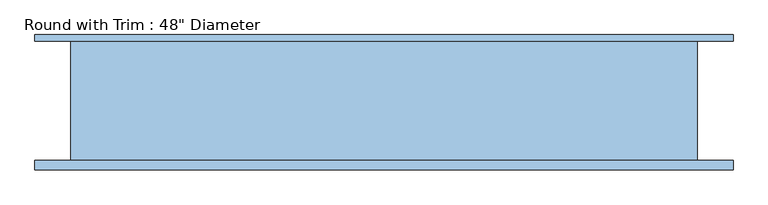
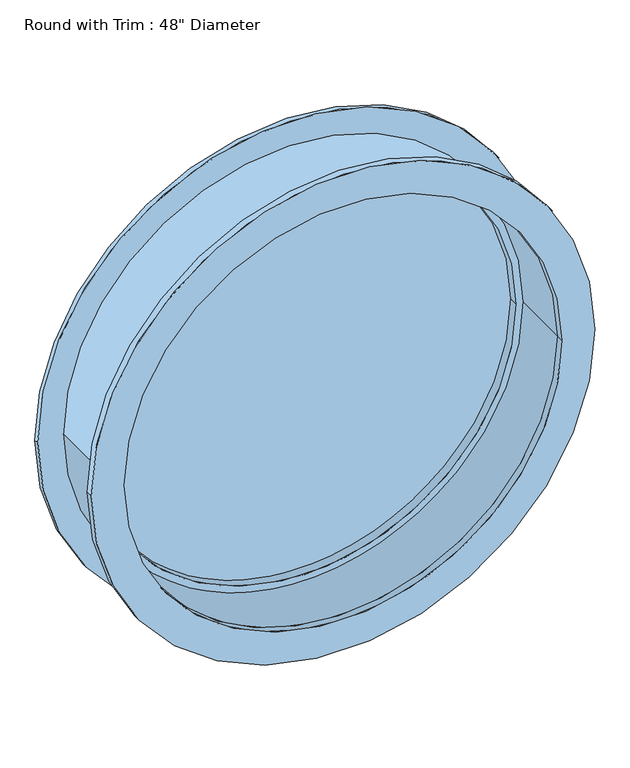
"""IFC4 building model written with IfcOpenShell, lengths in millimetres: window geometry."""

import ifcopenshell
import ifcopenshell.guid

model = None  # the IFC model being written
_history = None  # IfcOwnerHistory: only IFC2X3 demands one
_inside = {}  # id of a spatial element -> (the spatial element, [elements in it])
_under = {}  # id of a project, library or spatial element -> (it, [spatial elements below it])
_declared = {}  # id of a project -> (the project, [libraries it declares])
_typed = {}  # id of a type object -> (the type object, [elements of that type])
_made_of = {}  # id of a material, layer set ... -> (it, [elements and type objects made of it])


def new_model(schema):
    """Start an empty IFC model of exactly this schema.

    Asked for "IFC4X3", IfcOpenShell would pick the latest addendum, in which some entities
    have other attributes; the version numbers below select the first issue.
    IFC2X3 requires an IfcOwnerHistory on every rooted entity: one is made here for all.
    """
    global model, _history
    if schema == "IFC4X3":
        model = ifcopenshell.file(schema_version=(4, 3, 0, 0))
    else:
        model = ifcopenshell.file(schema=schema)
    _inside.clear()
    _under.clear()
    _declared.clear()
    _typed.clear()
    _made_of.clear()
    _history = None
    if model.schema == "IFC2X3":
        org = make("IfcOrganization", Name="unknown")
        user = make(
            "IfcPersonAndOrganization",
            ThePerson=make("IfcPerson", FamilyName="unknown"),
            TheOrganization=org,
        )
        app = make(
            "IfcApplication",
            ApplicationDeveloper=org,
            Version="unknown",
            ApplicationFullName="unknown",
            ApplicationIdentifier="unknown",
        )
        _history = make(
            "IfcOwnerHistory",
            OwningUser=user,
            OwningApplication=app,
            ChangeAction="ADDED",
            CreationDate=0,
        )
    return model


def make(cls, **values):
    """One entity of the class cls with the attributes given. An attribute that is None is left unset."""
    return model.create_entity(
        cls, **{name: value for name, value in values.items() if value is not None}
    )


def rooted(cls, **values):
    """An entity with a GlobalId (a new one), such as an element, a storey or a relation."""
    return make(cls, GlobalId=ifcopenshell.guid.new(), OwnerHistory=_history, **values)


def si_unit(unit_type, name, prefix=None):
    """IfcSIUnit, for example si_unit("LENGTHUNIT", "METRE", prefix="MILLI")."""
    return make("IfcSIUnit", UnitType=unit_type, Prefix=prefix, Name=name)


def assignment(units):
    """IfcUnitAssignment: the units of a project."""
    return None if units is None else make("IfcUnitAssignment", Units=units)


def point(xyz):
    """IfcCartesianPoint."""
    return None if xyz is None else make("IfcCartesianPoint", Coordinates=xyz)


def direction(xyz):
    """IfcDirection."""
    return None if xyz is None else make("IfcDirection", DirectionRatios=xyz)


def frame(location, z_axis=None, x_axis=None):
    """IfcAxis2Placement3D, a coordinate frame: its origin and axes. An axis left out is left unset."""
    return make(
        "IfcAxis2Placement3D",
        Location=point(location),
        Axis=direction(z_axis),
        RefDirection=direction(x_axis),
    )


def frame_2d(location, x_axis=None):
    """IfcAxis2Placement2D, a coordinate frame in the plane: its origin and x axis."""
    return make(
        "IfcAxis2Placement2D", Location=point(location), RefDirection=direction(x_axis)
    )


def origin():
    """The frame at (0, 0, 0) with its axes left unset."""
    return frame((0.0, 0.0, 0.0))


def place(relative_to, where):
    """IfcLocalPlacement: puts the frame where relative to a parent placement (None: the world)."""
    return make(
        "IfcLocalPlacement", PlacementRelTo=relative_to, RelativePlacement=where
    )


def context(
    kind, dimensions, precision=None, world=None, true_north=None, identifier=None
):
    """IfcGeometricRepresentationContext, for example the 3D "Model" context."""
    return make(
        "IfcGeometricRepresentationContext",
        ContextIdentifier=identifier,
        ContextType=kind,
        CoordinateSpaceDimension=dimensions,
        Precision=precision,
        WorldCoordinateSystem=world,
        TrueNorth=true_north,
    )


def project(units=None, contexts=None):
    """IfcProject with its units and contexts."""
    return rooted(
        "IfcProject",
        Name="project",
        RepresentationContexts=contexts,
        UnitsInContext=assignment(units),
    )


def spatial(cls, under=None, at=None, **own):
    """A site, building, storey or space (cls), placed at a placement, below another one or the project."""
    s = rooted(cls, ObjectPlacement=at, **own)
    if under is not None:
        _under.setdefault(under.id(), (under, []))[1].append(s)
    return s


def circle_curve(where, radius):
    """IfcCircle in the frame where."""
    return make("IfcCircle", Position=where, Radius=radius)


def trimmed(basis, trim1, trim2, sense, master):
    """IfcTrimmedCurve: the piece of a basis curve between two trims."""
    return make(
        "IfcTrimmedCurve",
        BasisCurve=basis,
        Trim1=trim1,
        Trim2=trim2,
        SenseAgreement=sense,
        MasterRepresentation=master,
    )


def segment(curve, same_sense, transition):
    """IfcCompositeCurveSegment."""
    return make(
        "IfcCompositeCurveSegment",
        Transition=transition,
        SameSense=same_sense,
        ParentCurve=curve,
    )


def composite_curve(segments, self_intersect=None):
    """IfcCompositeCurve: segments joined end to end."""
    return make("IfcCompositeCurve", Segments=segments, SelfIntersect=self_intersect)


def outline(outer, holes=None, kind="AREA"):
    """IfcArbitraryClosedProfileDef: a profile drawn as a closed curve; with holes, ...WithVoids."""
    if holes is None:
        return make("IfcArbitraryClosedProfileDef", ProfileType=kind, OuterCurve=outer)
    return make(
        "IfcArbitraryProfileDefWithVoids",
        ProfileType=kind,
        OuterCurve=outer,
        InnerCurves=holes,
    )


def extrude(swept, where, along, depth):
    """IfcExtrudedAreaSolid: the profile swept, set in the frame where, extruded along a direction by depth."""
    return make(
        "IfcExtrudedAreaSolid",
        SweptArea=swept,
        Position=where,
        ExtrudedDirection=direction(along),
        Depth=depth,
    )


def shape(context_of_items, identifier, shape_type, items):
    """IfcShapeRepresentation: the items that make up one representation, for example the "Body"."""
    return make(
        "IfcShapeRepresentation",
        ContextOfItems=context_of_items,
        RepresentationIdentifier=identifier,
        RepresentationType=shape_type,
        Items=items,
    )


def source(mapping_origin, context_of_items, identifier, shape_type, items):
    """IfcRepresentationMap: a shape defined once, which mapped items show again and again."""
    return make(
        "IfcRepresentationMap",
        MappingOrigin=mapping_origin,
        MappedRepresentation=shape(context_of_items, identifier, shape_type, items),
    )


def transform(
    local_origin,
    x_axis=None,
    y_axis=None,
    z_axis=None,
    scale=None,
    scale2=None,
    scale3=None,
    uniform=True,
):
    """IfcCartesianTransformationOperator3D, or its non-uniform kind. x_axis, y_axis, z_axis: its Axis1, 2, 3."""
    if uniform:
        return make(
            "IfcCartesianTransformationOperator3D",
            Axis1=direction(x_axis),
            Axis2=direction(y_axis),
            LocalOrigin=point(local_origin),
            Scale=scale,
            Axis3=direction(z_axis),
        )
    return make(
        "IfcCartesianTransformationOperator3DnonUniform",
        Axis1=direction(x_axis),
        Axis2=direction(y_axis),
        LocalOrigin=point(local_origin),
        Scale=scale,
        Axis3=direction(z_axis),
        Scale2=scale2,
        Scale3=scale3,
    )


def mapped(mapping_source, mapping_target):
    """IfcMappedItem: shows the shape of a source again, moved by a transform."""
    return make(
        "IfcMappedItem", MappingSource=mapping_source, MappingTarget=mapping_target
    )


def made_of(thing, what):
    """Note that an element or type object is made of a material, layer set ...; save() writes the relation."""
    if what is not None:
        _made_of.setdefault(what.id(), (what, []))[1].append(thing)
    return thing


def element(
    cls,
    number,
    at=None,
    inside=None,
    cuts=None,
    type_object=None,
    material=None,
    context=None,
    identifier="Body",
    shape_type=None,
    held_by="IfcProductDefinitionShape",
    body=None,
    shapes=None,
    **own,
):
    """One element of the class cls, such as IfcWall. Its Tag is "e" and its number.

    at: its placement. inside: the storey or other place that contains it. cuts: it is an
    opening in that element (IfcRelVoidsElement). A single representation is given by context,
    identifier, shape_type and body (its items); several are given by shapes. held_by: the class
    of the entity that holds the representations. save() writes the other relations.
    """
    e = rooted(cls, Tag="e%d" % number, ObjectPlacement=at, **own)
    if body is not None:
        shapes = [shape(context, identifier, shape_type, body)]
    if shapes is not None:
        e.Representation = make(held_by, Representations=shapes)
    if inside is not None:
        _inside.setdefault(inside.id(), (inside, []))[1].append(e)
    if cuts is not None:
        rooted(
            "IfcRelVoidsElement", RelatingBuildingElement=cuts, RelatedOpeningElement=e
        )
    if type_object is not None:
        _typed.setdefault(type_object.id(), (type_object, []))[1].append(e)
    return made_of(e, material)


def aggregate(whole, parts):
    """IfcRelAggregates: a whole, such as a stair, and the parts it consists of."""
    return rooted("IfcRelAggregates", RelatingObject=whole, RelatedObjects=parts)


def save(model, path):
    """Write the relations noted so far, then the file.

    IfcRelAggregates (storeys below a building ...), IfcRelContainedInSpatialStructure (elements
    in a storey), IfcRelDefinesByType, IfcRelAssociatesMaterial and IfcRelDeclares: one each for
    every whole, place, type object, material and project.
    """
    for whole, parts in _under.values():
        aggregate(whole, parts)
    for where, things in _inside.values():
        rooted(
            "IfcRelContainedInSpatialStructure",
            RelatedElements=things,
            RelatingStructure=where,
        )
    for kind, things in _typed.values():
        rooted("IfcRelDefinesByType", RelatedObjects=things, RelatingType=kind)
    for what, things in _made_of.values():
        rooted("IfcRelAssociatesMaterial", RelatedObjects=things, RelatingMaterial=what)
    for by, libraries in _declared.values():
        rooted("IfcRelDeclares", RelatingContext=by, RelatedDefinitions=libraries)
    model.write(path)


def window_c0979b06(model_context):
    return source(origin(), model_context, "Body", "SweptSolid", [
        extrude(outline(composite_curve([segment(trimmed(circle_curve(frame_2d((1219.2, 152.4)), 679.45), [point((1219.2, -527.05))], [point((1219.2, 831.85))], False, "CARTESIAN"), True, "CONTINUOUS"), segment(trimmed(circle_curve(frame_2d((1219.2, 152.4)), 679.45), [point((1219.2, 831.85))], [point((1219.2, -527.05))], False, "CARTESIAN"), True, "CONTINUOUS")], self_intersect=False), holes=[composite_curve([segment(trimmed(circle_curve(frame_2d((1219.2, 152.4)), 590.55), [point((1219.2, -438.15))], [point((1219.2, 742.95))], True, "CARTESIAN"), True, "CONTINUOUS"), segment(trimmed(circle_curve(frame_2d((1219.2, 152.4)), 590.55), [point((1219.2, 742.95))], [point((1219.2, -438.15))], True, "CARTESIAN"), True, "CONTINUOUS")], self_intersect=False)]), frame((0.0, -134.9375008, 0.0), z_axis=(0.0, 1.0, 0.0), x_axis=(0.0, 0.0, 1.0)), (0.0, 0.0, 1.0), 19.05),
        extrude(outline(composite_curve([segment(trimmed(circle_curve(frame_2d((1219.2, 152.4)), 679.45), [point((1219.2, -527.05))], [point((1219.2, 831.85))], False, "CARTESIAN"), True, "CONTINUOUS"), segment(trimmed(circle_curve(frame_2d((1219.2, 152.4)), 679.45), [point((1219.2, 831.85))], [point((1219.2, -527.05))], False, "CARTESIAN"), True, "CONTINUOUS")], self_intersect=False), holes=[composite_curve([segment(trimmed(circle_curve(frame_2d((1219.2, 152.4)), 590.55), [point((1219.2, -438.15))], [point((1219.2, 742.95))], True, "CARTESIAN"), True, "CONTINUOUS"), segment(trimmed(circle_curve(frame_2d((1219.2, 152.4)), 590.55), [point((1219.2, 742.95))], [point((1219.2, -438.15))], True, "CARTESIAN"), True, "CONTINUOUS")], self_intersect=False)]), frame((0.0, 115.8875008, 0.0), z_axis=(0.0, 1.0, 0.0), x_axis=(0.0, 0.0, 1.0)), (0.0, 0.0, 1.0), 12.7),
        extrude(outline(composite_curve([segment(trimmed(circle_curve(frame_2d((1219.2, 152.4)), 571.5), [point((1219.2, -419.1))], [point((1219.2, 723.9))], False, "CARTESIAN"), True, "CONTINUOUS"), segment(trimmed(circle_curve(frame_2d((1219.2, 152.4)), 571.5), [point((1219.2, 723.9))], [point((1219.2, -419.1))], False, "CARTESIAN"), True, "CONTINUOUS")], self_intersect=False)), frame((0.0, 71.4375008, 0.0), z_axis=(0.0, 1.0, 0.0), x_axis=(0.0, 0.0, 1.0)), (0.0, 0.0, 1.0), 12.7),
        extrude(outline(composite_curve([segment(trimmed(circle_curve(frame_2d((1219.2, 152.4)), 590.55), [point((1219.2, -438.15))], [point((1219.2, 742.95))], False, "CARTESIAN"), True, "CONTINUOUS"), segment(trimmed(circle_curve(frame_2d((1219.2, 152.4)), 590.55), [point((1219.2, 742.95))], [point((1219.2, -438.15))], False, "CARTESIAN"), True, "CONTINUOUS")], self_intersect=False), holes=[composite_curve([segment(trimmed(circle_curve(frame_2d((1219.2, 152.4)), 571.5), [point((1219.2, -419.1))], [point((1219.2, 723.9))], True, "CARTESIAN"), True, "CONTINUOUS"), segment(trimmed(circle_curve(frame_2d((1219.2, 152.4)), 571.5), [point((1219.2, 723.9))], [point((1219.2, -419.1))], True, "CARTESIAN"), True, "CONTINUOUS")], self_intersect=False)]), frame((0.0, 46.0375008, 0.0), z_axis=(0.0, 1.0, 0.0), x_axis=(0.0, 0.0, 1.0)), (0.0, 0.0, 1.0), 50.8),
        extrude(outline(composite_curve([segment(trimmed(circle_curve(frame_2d((1219.2, 152.4)), 609.6), [point((1219.2, -457.2))], [point((1219.2, 762.0))], False, "CARTESIAN"), True, "CONTINUOUS"), segment(trimmed(circle_curve(frame_2d((1219.2, 152.4)), 609.6), [point((1219.2, 762.0))], [point((1219.2, -457.2))], False, "CARTESIAN"), True, "CONTINUOUS")], self_intersect=False), holes=[composite_curve([segment(trimmed(circle_curve(frame_2d((1219.2, 152.4)), 590.55), [point((1219.2, -438.15))], [point((1219.2, 742.95))], True, "CARTESIAN"), True, "CONTINUOUS"), segment(trimmed(circle_curve(frame_2d((1219.2, 152.4)), 590.55), [point((1219.2, 742.95))], [point((1219.2, -438.15))], True, "CARTESIAN"), True, "CONTINUOUS")], self_intersect=False)]), frame((0.0, -115.8875008, 0.0), z_axis=(0.0, 1.0, 0.0), x_axis=(0.0, 0.0, 1.0)), (0.0, 0.0, 1.0), 231.7750015),
    ])


if __name__ == "__main__":
    model = new_model("IFC4")
    model_context = context("Model", 3, world=origin())
    ifc_project = project(units=[si_unit("LENGTHUNIT", "METRE", prefix="MILLI")], contexts=[model_context])
    site = spatial("IfcSite", under=ifc_project)
    building = spatial("IfcBuilding", under=site)
    placement = place(None, origin())
    window_shape = window_c0979b06(model_context)
    element("IfcWindow", 1, ObjectType="Round with Trim : 48\" Diameter", at=placement, inside=building, context=model_context, shape_type="MappedRepresentation", body=[
        mapped(window_shape, transform((0.0, 0.0, 0.0), x_axis=(1.0, 0.0, 0.0), y_axis=(0.0, 1.0, 0.0), z_axis=(0.0, 0.0, 1.0))),
    ])
    save(model, "model.ifc")

# Revit data of these elements
# Type "Round with Trim : 48\" Diameter"
#   Type Mark = "26"
#   COBie.Type.CreatedBy = "doug.wood@us.ibm.com"
#   COBie.Type.CreatedOn = "2016-04-14T02:07:26"
#   COBie.Type.Name = "Windows_Round with Trim_48\" Diameter_26"
#   COBie.Type.Category = "23-30 20 00 : Windows"
#   COBie.Type.Description = "Round with Trim_48\" Diameter"
#   COBie.Type.Manufacturer = ""
#   COBie.Type.ModelNumber = ""
#   Construction Type Id = "GSP4R"
#   Assembly Code = "B2020100"
#   Analytic Construction = "1/8 in Pilkington single glazing"
#   COBie.Type.ReplacementCost = 0
#   Visual Light Transmittance = 0.9
#   Solar Heat Gain Coefficient = 0.78
#   Heat Transfer Coefficient (U) = 3.6886 W/(m²·K)
#   Default Sill Height = 2' - 0"
#   Trim Projection - Ext. = 0' - 0 1/2"
#   Trim Projection - Int. = 0' - 0 3/4"
#   Trim Width - Exterior = 0' - 3 1/2"
#   Trim Width - Interior = 0' - 3 1/2"
#   Width = 4' - 0"
#   COBie.Type = no
#   Glass Pane Material = Glass
#   Sash Material = Sash - White
#   Trim Exterior Material = Trim - White
#   Trim Interior Material = Trim - White
#   Wall Closure = (empty or 0)
# Element 1 (IfcWindow, "Round with Trim : 48\" Diameter")
#   Materials on its faces: "Trim - White", "Sash - White", "Glass"
# Materials
#   "Glass": class "Glass", colour RGB 0 128 192, transparency 0.75, Description = "Soda Lime Glass", Cost = 0
#   "Sash - White": class "Wood", colour RGB 255 255 255, transparency 0, Cost = 0
#   "Trim - White": class "Wood", colour RGB 255 255 255, transparency 0, Cost = 0
